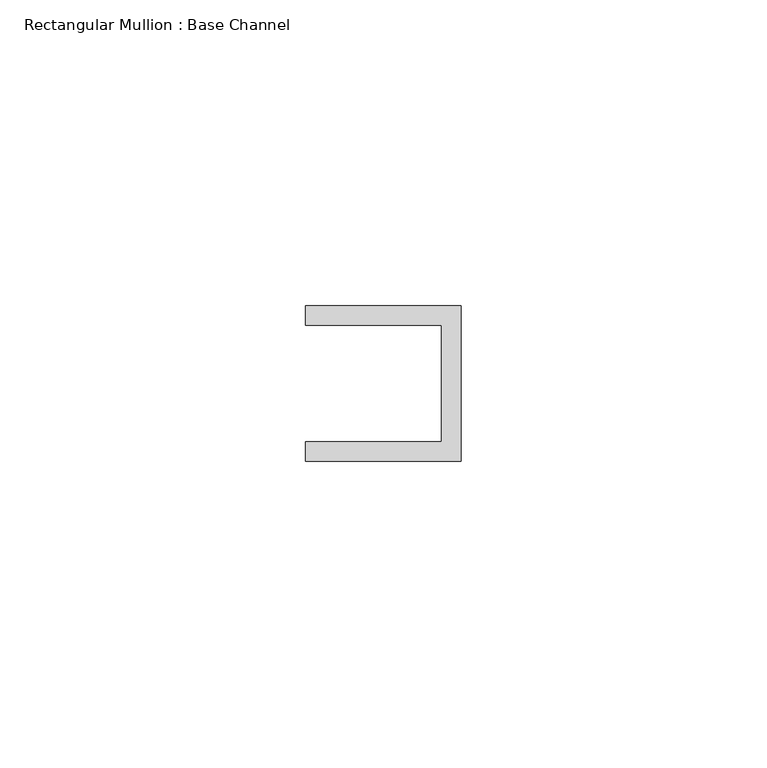
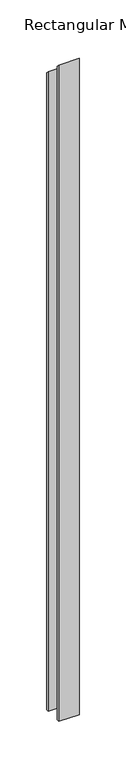
"""IFC4 building model written with IfcOpenShell, lengths in millimetres: member geometry, Rectangular Mullion : Base Channel."""

from ifc_helpers import new_model, si_unit, origin, place, context, project, spatial, faceted_brep, source, transform, mapped, element, save


def rectangular_mullion_base_channel_f724732a(model_context):
    return source(origin(), model_context, "Body", "Brep", [
        faceted_brep([(0.0, -12.7, -845.4185498), (-25.4, -12.7, -845.4185498), (-25.4, -9.525, -845.4185498), (-3.175, -9.525, -845.4185498), (-3.175, 9.525, -845.4185498), (-25.4, 9.525, -845.4185498), (-25.4, 12.7, -845.4185498), (0.0, 12.7, -845.4185498), (0.0, 12.7, -12.7), (0.0, -12.7, 12.7), (-25.4, 12.7, -12.7), (-25.4, 9.525, -9.525), (-3.175, 9.525, -9.525), (-3.175, -9.525, 9.525), (-25.4, -9.525, 9.525), (-25.4, -12.7, 12.7)], [[[0, 1, 2, 3, 4, 5, 6, 7]], [[8, 9, 0, 7]], [[10, 8, 7, 6]], [[11, 10, 6, 5]], [[12, 11, 5, 4]], [[13, 12, 4, 3]], [[14, 13, 3, 2]], [[15, 14, 2, 1]], [[9, 15, 1, 0]], [[9, 8, 10, 11, 12, 13, 14, 15]]]),
    ])


if __name__ == "__main__":
    model = new_model("IFC4")
    model_context = context("Model", 3, world=origin())
    ifc_project = project(units=[si_unit("LENGTHUNIT", "METRE", prefix="MILLI")], contexts=[model_context])
    site = spatial("IfcSite", under=ifc_project)
    building = spatial("IfcBuilding", under=site)
    placement = place(None, origin())
    rectangular_mullion_base_channel_shape = rectangular_mullion_base_channel_f724732a(model_context)
    element("IfcMember", 1, ObjectType="Rectangular Mullion : Base Channel", at=placement, inside=building, context=model_context, shape_type="MappedRepresentation", body=[
        mapped(rectangular_mullion_base_channel_shape, transform((0.0, 0.0, 0.0), x_axis=(1.0, 0.0, 0.0), y_axis=(0.0, 1.0, 0.0), z_axis=(0.0, 0.0, 1.0))),
    ])
    save(model, "model.ifc")

# Revit data of these elements
# Type "Rectangular Mullion : Base Channel"
#   built-in parameter 1007322 = 0.0833333 (stored number, unit not read)
#   built-in parameter 1007321 = 0.0416667 (stored number, unit not read)
#   built-in parameter 1007320 = -0.03125 (stored number, unit not read)
# Element 1 (IfcMember, "Rectangular Mullion : Base Channel")
#   Materials on its faces: "ALUM"
# Materials
#   "ALUM": class "Generic", colour RGB 157 157 157, transparency 0, Cost = 0
